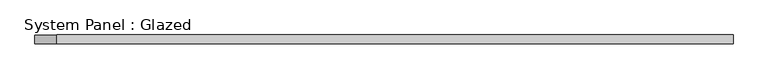
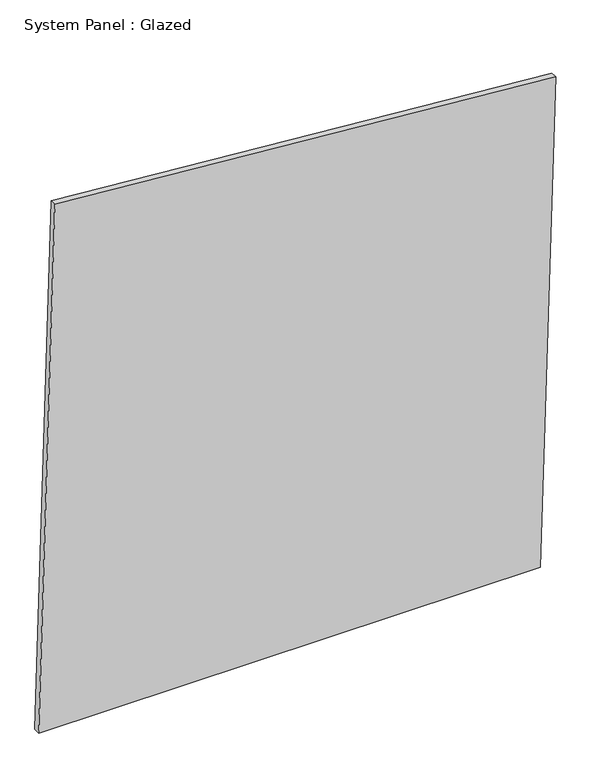
"""IFC4 building model written with IfcOpenShell, lengths in millimetres: plate geometry, System Panel : Glazed."""

from ifc_helpers import new_model, si_unit, frame, origin, place, context, project, spatial, polyline, outline, extrude, source, transform, mapped, element, save


def system_panel_glazed_cfa6e621(model_context):
    return source(origin(), model_context, "Body", "SweptSolid", [
        extrude(outline(polyline([(0.0, -1005.3178204), (0.0, 944.6224941), (1993.8665555, 1005.3178204), (2151.1709359, -942.2983527), (0.0, -1005.3178204)])), frame((0.0, -49.5, 0.0), z_axis=(0.0, 1.0, 0.0), x_axis=(0.0, 0.0, 1.0)), (0.0, 0.0, 1.0), 25.0),
    ])


if __name__ == "__main__":
    model = new_model("IFC4")
    model_context = context("Model", 3, world=origin())
    ifc_project = project(units=[si_unit("LENGTHUNIT", "METRE", prefix="MILLI")], contexts=[model_context])
    site = spatial("IfcSite", under=ifc_project)
    building = spatial("IfcBuilding", under=site)
    placement = place(None, origin())
    system_panel_glazed_shape = system_panel_glazed_cfa6e621(model_context)
    element("IfcPlate", 1, ObjectType="System Panel : Glazed", at=placement, inside=building, context=model_context, shape_type="MappedRepresentation", body=[
        mapped(system_panel_glazed_shape, transform((0.0, 0.0, 0.0), x_axis=(1.0, 0.0, 0.0), y_axis=(0.0, 1.0, 0.0), z_axis=(0.0, 0.0, 1.0))),
    ])
    save(model, "model.ifc")

# Revit data of these elements
# Element 1 (IfcPlate, "System Panel : Glazed")
#   Materials on its faces: "Glass, Clear Glazing"
# Materials
#   "Glass, Clear Glazing": class "Glass", colour RGB 247 249 248, transparency 0.85, Description = "Clear glazing", Cost = 0
